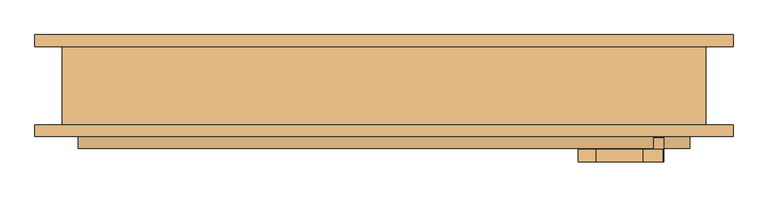
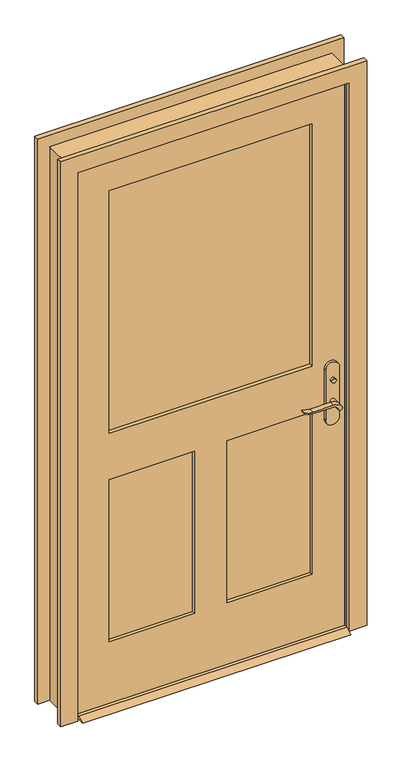
"""IFC4 building model written with IfcOpenShell, lengths in millimetres: door geometry."""

import ifcopenshell
import ifcopenshell.guid

model = None  # the IFC model being written
_history = None  # IfcOwnerHistory: only IFC2X3 demands one
_inside = {}  # id of a spatial element -> (the spatial element, [elements in it])
_under = {}  # id of a project, library or spatial element -> (it, [spatial elements below it])
_declared = {}  # id of a project -> (the project, [libraries it declares])
_typed = {}  # id of a type object -> (the type object, [elements of that type])
_made_of = {}  # id of a material, layer set ... -> (it, [elements and type objects made of it])


def new_model(schema):
    """Start an empty IFC model of exactly this schema.

    Asked for "IFC4X3", IfcOpenShell would pick the latest addendum, in which some entities
    have other attributes; the version numbers below select the first issue.
    IFC2X3 requires an IfcOwnerHistory on every rooted entity: one is made here for all.
    """
    global model, _history
    if schema == "IFC4X3":
        model = ifcopenshell.file(schema_version=(4, 3, 0, 0))
    else:
        model = ifcopenshell.file(schema=schema)
    _inside.clear()
    _under.clear()
    _declared.clear()
    _typed.clear()
    _made_of.clear()
    _history = None
    if model.schema == "IFC2X3":
        org = make("IfcOrganization", Name="unknown")
        user = make(
            "IfcPersonAndOrganization",
            ThePerson=make("IfcPerson", FamilyName="unknown"),
            TheOrganization=org,
        )
        app = make(
            "IfcApplication",
            ApplicationDeveloper=org,
            Version="unknown",
            ApplicationFullName="unknown",
            ApplicationIdentifier="unknown",
        )
        _history = make(
            "IfcOwnerHistory",
            OwningUser=user,
            OwningApplication=app,
            ChangeAction="ADDED",
            CreationDate=0,
        )
    return model


def make(cls, **values):
    """One entity of the class cls with the attributes given. An attribute that is None is left unset."""
    return model.create_entity(
        cls, **{name: value for name, value in values.items() if value is not None}
    )


def rooted(cls, **values):
    """An entity with a GlobalId (a new one), such as an element, a storey or a relation."""
    return make(cls, GlobalId=ifcopenshell.guid.new(), OwnerHistory=_history, **values)


def si_unit(unit_type, name, prefix=None):
    """IfcSIUnit, for example si_unit("LENGTHUNIT", "METRE", prefix="MILLI")."""
    return make("IfcSIUnit", UnitType=unit_type, Prefix=prefix, Name=name)


def assignment(units):
    """IfcUnitAssignment: the units of a project."""
    return None if units is None else make("IfcUnitAssignment", Units=units)


def point(xyz):
    """IfcCartesianPoint."""
    return None if xyz is None else make("IfcCartesianPoint", Coordinates=xyz)


def direction(xyz):
    """IfcDirection."""
    return None if xyz is None else make("IfcDirection", DirectionRatios=xyz)


def frame(location, z_axis=None, x_axis=None):
    """IfcAxis2Placement3D, a coordinate frame: its origin and axes. An axis left out is left unset."""
    return make(
        "IfcAxis2Placement3D",
        Location=point(location),
        Axis=direction(z_axis),
        RefDirection=direction(x_axis),
    )


def frame_2d(location, x_axis=None):
    """IfcAxis2Placement2D, a coordinate frame in the plane: its origin and x axis."""
    return make(
        "IfcAxis2Placement2D", Location=point(location), RefDirection=direction(x_axis)
    )


def origin():
    """The frame at (0, 0, 0) with its axes left unset."""
    return frame((0.0, 0.0, 0.0))


def place(relative_to, where):
    """IfcLocalPlacement: puts the frame where relative to a parent placement (None: the world)."""
    return make(
        "IfcLocalPlacement", PlacementRelTo=relative_to, RelativePlacement=where
    )


def context(
    kind, dimensions, precision=None, world=None, true_north=None, identifier=None
):
    """IfcGeometricRepresentationContext, for example the 3D "Model" context."""
    return make(
        "IfcGeometricRepresentationContext",
        ContextIdentifier=identifier,
        ContextType=kind,
        CoordinateSpaceDimension=dimensions,
        Precision=precision,
        WorldCoordinateSystem=world,
        TrueNorth=true_north,
    )


def project(units=None, contexts=None):
    """IfcProject with its units and contexts."""
    return rooted(
        "IfcProject",
        Name="project",
        RepresentationContexts=contexts,
        UnitsInContext=assignment(units),
    )


def spatial(cls, under=None, at=None, **own):
    """A site, building, storey or space (cls), placed at a placement, below another one or the project."""
    s = rooted(cls, ObjectPlacement=at, **own)
    if under is not None:
        _under.setdefault(under.id(), (under, []))[1].append(s)
    return s


def polyline(points):
    """IfcPolyline through the points."""
    return make("IfcPolyline", Points=[point(p) for p in points])


def circle_curve(where, radius):
    """IfcCircle in the frame where."""
    return make("IfcCircle", Position=where, Radius=radius)


def trimmed(basis, trim1, trim2, sense, master):
    """IfcTrimmedCurve: the piece of a basis curve between two trims."""
    return make(
        "IfcTrimmedCurve",
        BasisCurve=basis,
        Trim1=trim1,
        Trim2=trim2,
        SenseAgreement=sense,
        MasterRepresentation=master,
    )


def segment(curve, same_sense, transition):
    """IfcCompositeCurveSegment."""
    return make(
        "IfcCompositeCurveSegment",
        Transition=transition,
        SameSense=same_sense,
        ParentCurve=curve,
    )


def composite_curve(segments, self_intersect=None):
    """IfcCompositeCurve: segments joined end to end."""
    return make("IfcCompositeCurve", Segments=segments, SelfIntersect=self_intersect)


def outline(outer, holes=None, kind="AREA"):
    """IfcArbitraryClosedProfileDef: a profile drawn as a closed curve; with holes, ...WithVoids."""
    if holes is None:
        return make("IfcArbitraryClosedProfileDef", ProfileType=kind, OuterCurve=outer)
    return make(
        "IfcArbitraryProfileDefWithVoids",
        ProfileType=kind,
        OuterCurve=outer,
        InnerCurves=holes,
    )


def extrude(swept, where, along, depth):
    """IfcExtrudedAreaSolid: the profile swept, set in the frame where, extruded along a direction by depth."""
    return make(
        "IfcExtrudedAreaSolid",
        SweptArea=swept,
        Position=where,
        ExtrudedDirection=direction(along),
        Depth=depth,
    )


def faces_of(points, faces, orient=None, outer=None):
    """IfcFace entities. A face is a list of loops; a loop is a list of indices into points, from 0.

    orient and outer hold one flag for each loop. By default every Orientation is true, the
    first loop of a face is its IfcFaceOuterBound and the others are IfcFaceBound.
    """
    made = []
    for i, loops in enumerate(faces):
        bounds = []
        for j, loop in enumerate(loops):
            is_outer = j == 0 if outer is None else outer[i][j]
            bounds.append(
                make(
                    "IfcFaceOuterBound" if is_outer else "IfcFaceBound",
                    Bound=make("IfcPolyLoop", Polygon=[points[k] for k in loop]),
                    Orientation=True if orient is None else orient[i][j],
                )
            )
        made.append(make("IfcFace", Bounds=bounds))
    return made


def faceted_brep(points, faces, orient=None, outer=None, voids=None):
    """IfcFacetedBrep: a solid bounded by flat faces; with voids (closed shells), ...WithVoids."""
    shared = [point(p) for p in points]
    hull = make("IfcClosedShell", CfsFaces=faces_of(shared, faces, orient, outer))
    if voids is None:
        return make("IfcFacetedBrep", Outer=hull)
    return make(
        "IfcFacetedBrepWithVoids",
        Outer=hull,
        Voids=[
            make(cls, CfsFaces=faces_of(shared, fs, o, b)) for cls, fs, o, b in voids
        ],
    )


def shape(context_of_items, identifier, shape_type, items):
    """IfcShapeRepresentation: the items that make up one representation, for example the "Body"."""
    return make(
        "IfcShapeRepresentation",
        ContextOfItems=context_of_items,
        RepresentationIdentifier=identifier,
        RepresentationType=shape_type,
        Items=items,
    )


def source(mapping_origin, context_of_items, identifier, shape_type, items):
    """IfcRepresentationMap: a shape defined once, which mapped items show again and again."""
    return make(
        "IfcRepresentationMap",
        MappingOrigin=mapping_origin,
        MappedRepresentation=shape(context_of_items, identifier, shape_type, items),
    )


def transform(
    local_origin,
    x_axis=None,
    y_axis=None,
    z_axis=None,
    scale=None,
    scale2=None,
    scale3=None,
    uniform=True,
):
    """IfcCartesianTransformationOperator3D, or its non-uniform kind. x_axis, y_axis, z_axis: its Axis1, 2, 3."""
    if uniform:
        return make(
            "IfcCartesianTransformationOperator3D",
            Axis1=direction(x_axis),
            Axis2=direction(y_axis),
            LocalOrigin=point(local_origin),
            Scale=scale,
            Axis3=direction(z_axis),
        )
    return make(
        "IfcCartesianTransformationOperator3DnonUniform",
        Axis1=direction(x_axis),
        Axis2=direction(y_axis),
        LocalOrigin=point(local_origin),
        Scale=scale,
        Axis3=direction(z_axis),
        Scale2=scale2,
        Scale3=scale3,
    )


def mapped(mapping_source, mapping_target):
    """IfcMappedItem: shows the shape of a source again, moved by a transform."""
    return make(
        "IfcMappedItem", MappingSource=mapping_source, MappingTarget=mapping_target
    )


def made_of(thing, what):
    """Note that an element or type object is made of a material, layer set ...; save() writes the relation."""
    if what is not None:
        _made_of.setdefault(what.id(), (what, []))[1].append(thing)
    return thing


def element(
    cls,
    number,
    at=None,
    inside=None,
    cuts=None,
    type_object=None,
    material=None,
    context=None,
    identifier="Body",
    shape_type=None,
    held_by="IfcProductDefinitionShape",
    body=None,
    shapes=None,
    **own,
):
    """One element of the class cls, such as IfcWall. Its Tag is "e" and its number.

    at: its placement. inside: the storey or other place that contains it. cuts: it is an
    opening in that element (IfcRelVoidsElement). A single representation is given by context,
    identifier, shape_type and body (its items); several are given by shapes. held_by: the class
    of the entity that holds the representations. save() writes the other relations.
    """
    e = rooted(cls, Tag="e%d" % number, ObjectPlacement=at, **own)
    if body is not None:
        shapes = [shape(context, identifier, shape_type, body)]
    if shapes is not None:
        e.Representation = make(held_by, Representations=shapes)
    if inside is not None:
        _inside.setdefault(inside.id(), (inside, []))[1].append(e)
    if cuts is not None:
        rooted(
            "IfcRelVoidsElement", RelatingBuildingElement=cuts, RelatedOpeningElement=e
        )
    if type_object is not None:
        _typed.setdefault(type_object.id(), (type_object, []))[1].append(e)
    return made_of(e, material)


def aggregate(whole, parts):
    """IfcRelAggregates: a whole, such as a stair, and the parts it consists of."""
    return rooted("IfcRelAggregates", RelatingObject=whole, RelatedObjects=parts)


def save(model, path):
    """Write the relations noted so far, then the file.

    IfcRelAggregates (storeys below a building ...), IfcRelContainedInSpatialStructure (elements
    in a storey), IfcRelDefinesByType, IfcRelAssociatesMaterial and IfcRelDeclares: one each for
    every whole, place, type object, material and project.
    """
    for whole, parts in _under.values():
        aggregate(whole, parts)
    for where, things in _inside.values():
        rooted(
            "IfcRelContainedInSpatialStructure",
            RelatedElements=things,
            RelatingStructure=where,
        )
    for kind, things in _typed.values():
        rooted("IfcRelDefinesByType", RelatedObjects=things, RelatingType=kind)
    for what, things in _made_of.values():
        rooted("IfcRelAssociatesMaterial", RelatedObjects=things, RelatingMaterial=what)
    for by, libraries in _declared.values():
        rooted("IfcRelDeclares", RelatingContext=by, RelatedDefinitions=libraries)
    model.write(path)


def door_f2be2632(model_context):
    return source(origin(), model_context, "Body", "SolidModel", [
        extrude(outline(polyline([(-38.1, 12.7), (-12.7, 0.0), (-98.425, 0.0), (-73.025, 12.7), (-38.1, 12.7)])), frame((-495.3, 0.0, 0.0), z_axis=(1.0, 0.0, 0.0), x_axis=(0.0, 1.0, 0.0)), (0.0, 0.0, 1.0), 990.6),
        extrude(outline(polyline([(449.5, -5.4), (449.5, -15.4), (439.5, -15.4), (439.5, -5.4), (449.5, -5.4)])), frame((0.0, 0.0, 981.9), z_axis=(0.0, 0.0, 1.0), x_axis=(1.0, 0.0, 0.0)), (0.0, 0.0, 1.0), 30.0),
        extrude(outline(composite_curve([segment(trimmed(circle_curve(frame_2d((996.9, 444.5)), 8.0), [point((996.9, 436.5))], [point((996.9, 452.5))], False, "CARTESIAN"), True, "CONTINUOUS"), segment(trimmed(circle_curve(frame_2d((996.9, 444.5)), 8.0), [point((996.9, 452.5))], [point((996.9, 436.5))], False, "CARTESIAN"), True, "CONTINUOUS")], self_intersect=False)), frame((0.0, -80.325, 0.0), z_axis=(0.0, 1.0, 0.0), x_axis=(0.0, 0.0, 1.0)), (0.0, 0.0, 1.0), 10.0),
        extrude(outline(composite_curve([segment(trimmed(circle_curve(frame_2d((897.1555521, 420.8324871)), 37.2832219), [point((919.0523287, 451.0081363))], [point((934.4, 419.1325667))], False, "CARTESIAN"), True, "CONTINUOUS"), segment(polyline([(934.4, 419.1325667), (934.4, 342.8564091)]), True, "CONTINUOUS"), segment(trimmed(circle_curve(frame_2d((1017.6850638, 342.9227909)), 83.2850902), [point((934.4, 342.8564091))], [point((939.4, 314.5))], True, "CARTESIAN"), True, "CONTINUOUS"), segment(polyline([(939.4, 314.5), (936.6135558, 314.5)]), True, "CONTINUOUS"), segment(trimmed(circle_curve(frame_2d((986.6709207, 346.4396612)), 59.3791355), [point((936.6135558, 314.5))], [point((927.4, 342.8564091))], False, "CARTESIAN"), True, "CONTINUOUS"), segment(polyline([(927.4, 342.8564091), (927.4, 419.1138099)]), True, "CONTINUOUS"), segment(trimmed(circle_curve(frame_2d((909.2738613, 419.1138099)), 18.1261387), [point((927.4, 419.1138099))], [point((914.4, 436.5))], True, "CARTESIAN"), True, "CONTINUOUS"), segment(trimmed(circle_curve(frame_2d((914.4, 444.5)), 8.0), [point((914.4, 436.5))], [point((919.0523287, 451.0081363))], False, "CARTESIAN"), True, "CONTINUOUS")], self_intersect=False)), frame((0.0, 14.6, 0.0), z_axis=(0.0, 1.0, 0.0), x_axis=(0.0, 0.0, 1.0)), (0.0, 0.0, 1.0), 20.0),
        extrude(outline(composite_curve([segment(trimmed(circle_curve(frame_2d((914.4, 444.5)), 8.0), [point((914.3999903, 436.5))], [point((919.0523287, 451.0081363))], False, "CARTESIAN"), True, "CONTINUOUS"), segment(trimmed(circle_curve(frame_2d((897.1555521, 420.8324871)), 37.2832219), [point((919.0523287, 451.0081363))], [point((934.4, 419.1325667))], False, "CARTESIAN"), True, "CONTINUOUS"), segment(polyline([(934.4, 419.1325667), (934.4, 342.8564091)]), True, "CONTINUOUS"), segment(trimmed(circle_curve(frame_2d((1017.6850638, 342.9227909)), 83.2850902), [point((934.4, 342.8564091))], [point((939.4, 314.5))], True, "CARTESIAN"), True, "CONTINUOUS"), segment(polyline([(939.4, 314.5), (936.6135558, 314.5)]), True, "CONTINUOUS"), segment(trimmed(circle_curve(frame_2d((986.6709207, 346.4396612)), 59.3791355), [point((936.6135558, 314.5))], [point((927.4, 342.8564091))], False, "CARTESIAN"), True, "CONTINUOUS"), segment(polyline([(927.4, 342.8564091), (927.4, 419.1138122)]), True, "CONTINUOUS"), segment(trimmed(circle_curve(frame_2d((909.2738682, 419.1138122)), 18.1261318), [point((927.4, 419.1138122))], [point((914.3999903, 436.5))], True, "CARTESIAN"), True, "CONTINUOUS")], self_intersect=False)), frame((0.0, -120.325, 0.0), z_axis=(0.0, 1.0, 0.0), x_axis=(0.0, 0.0, 1.0)), (0.0, 0.0, 1.0), 20.0),
        extrude(outline(composite_curve([segment(trimmed(circle_curve(frame_2d((914.4, 444.5)), 8.0), [point((914.4, 436.5))], [point((914.4, 452.5))], False, "CARTESIAN"), True, "CONTINUOUS"), segment(trimmed(circle_curve(frame_2d((914.4, 444.5)), 8.0), [point((914.4, 452.5))], [point((914.4, 436.5))], False, "CARTESIAN"), True, "CONTINUOUS")], self_intersect=False)), frame((0.0, -15.4, 0.0), z_axis=(0.0, 1.0, 0.0), x_axis=(0.0, 0.0, 1.0)), (0.0, 0.0, 1.0), 30.0),
        extrude(outline(composite_curve([segment(trimmed(circle_curve(frame_2d((914.4, 444.5)), 8.0), [point((914.4, 436.5))], [point((914.4, 452.5))], False, "CARTESIAN"), True, "CONTINUOUS"), segment(trimmed(circle_curve(frame_2d((914.4, 444.5)), 8.0), [point((914.4, 452.5))], [point((914.4, 436.5))], False, "CARTESIAN"), True, "CONTINUOUS")], self_intersect=False)), frame((0.0, -100.325, 0.0), z_axis=(0.0, 1.0, 0.0), x_axis=(0.0, 0.0, 1.0)), (0.0, 0.0, 1.0), 30.0),
        extrude(outline(composite_curve([segment(polyline([(844.4, 469.5), (1039.4, 469.5)]), True, "CONTINUOUS"), segment(trimmed(circle_curve(frame_2d((1039.4, 444.5)), 25.0), [point((1039.4, 469.5))], [point((1039.4, 419.5))], False, "CARTESIAN"), True, "CONTINUOUS"), segment(polyline([(1039.4, 419.5), (844.4, 419.5)]), True, "CONTINUOUS"), segment(trimmed(circle_curve(frame_2d((844.4, 444.5)), 25.0), [point((844.4, 419.5))], [point((844.4, 469.5))], False, "CARTESIAN"), True, "CONTINUOUS")], self_intersect=False)), frame((0.0, -25.4, 0.0), z_axis=(0.0, 1.0, 0.0), x_axis=(0.0, 0.0, 1.0)), (0.0, 0.0, 1.0), 10.0),
        extrude(outline(composite_curve([segment(polyline([(844.4, 469.5), (1039.4, 469.5)]), True, "CONTINUOUS"), segment(trimmed(circle_curve(frame_2d((1039.4, 444.5)), 25.0), [point((1039.4, 469.5))], [point((1039.4, 419.5))], False, "CARTESIAN"), True, "CONTINUOUS"), segment(polyline([(1039.4, 419.5), (844.4, 419.5)]), True, "CONTINUOUS"), segment(trimmed(circle_curve(frame_2d((844.4, 444.5)), 25.0), [point((844.4, 419.5))], [point((844.4, 469.5))], False, "CARTESIAN"), True, "CONTINUOUS")], self_intersect=False)), frame((0.0, -70.325, 0.0), z_axis=(0.0, 1.0, 0.0), x_axis=(0.0, 0.0, 1.0)), (0.0, 0.0, 1.0), 10.0),
        faceted_brep([(520.7, -60.325, 0.0), (495.3, -60.325, 0.0), (495.3, -25.4, 0.0), (482.6, -25.4, 0.0), (482.6, 9.525, 0.0), (495.3, 9.525, 0.0), (495.3, 66.675, 0.0), (520.7, 66.675, 0.0), (520.7, 66.675, 2159.0), (520.7, -60.325, 2159.0), (495.3, 66.675, 2133.6), (-495.3, 66.675, 2133.6), (-495.3, 66.675, 0.0), (-520.7, 66.675, 0.0), (-520.7, 66.675, 2159.0), (495.3, 9.525, 2133.6), (482.6, 9.525, 2120.9), (-482.6, 9.525, 2120.9), (-482.6, 9.525, 0.0), (-495.3, 9.525, 0.0), (-495.3, 9.525, 2133.6), (482.6, -25.4, 2120.9), (495.3, -25.4, 2133.6), (-495.3, -25.4, 2133.6), (-495.3, -25.4, 0.0), (-482.6, -25.4, 0.0), (-482.6, -25.4, 2120.9), (495.3, -60.325, 2133.6), (-520.7, -60.325, 2159.0), (-520.7, -60.325, 0.0), (-495.3, -60.325, 0.0), (-495.3, -60.325, 2133.6)], [[[0, 1, 2, 3, 4, 5, 6, 7]], [[7, 8, 9, 0]], [[6, 10, 11, 12, 13, 14, 8, 7]], [[5, 15, 10, 6]], [[4, 16, 17, 18, 19, 20, 15, 5]], [[3, 21, 16, 4]], [[2, 22, 23, 24, 25, 26, 21, 3]], [[1, 27, 22, 2]], [[0, 9, 28, 29, 30, 31, 27, 1]], [[8, 14, 28, 9]], [[15, 20, 11, 10]], [[21, 26, 17, 16]], [[27, 31, 23, 22]], [[29, 13, 12, 19, 18, 25, 24, 30]], [[14, 13, 29, 28]], [[20, 19, 12, 11]], [[26, 25, 18, 17]], [[31, 30, 24, 23]]]),
        extrude(outline(polyline([(2133.6, -495.3), (12.7, -495.3), (12.7, 495.3), (2133.6, 495.3), (2133.6, -495.3)]), holes=[polyline([(1066.8, -374.65), (2012.95, -374.65), (2012.95, 374.65), (1066.8, 374.65), (1066.8, -374.65)]), polyline([(885.825, -60.325), (254.0, -60.325), (254.0, -374.65), (885.825, -374.65), (885.825, -60.325)]), polyline([(885.825, 374.65), (254.0, 374.65), (254.0, 60.325), (885.825, 60.325), (885.825, 374.65)])]), frame((0.0, -60.325, 0.0), z_axis=(0.0, 1.0, 0.0), x_axis=(0.0, 0.0, 1.0)), (0.0, 0.0, 1.0), 34.925),
        extrude(outline(polyline([(374.65, -39.37), (374.65, -46.355), (-374.65, -46.355), (-374.65, -39.37), (374.65, -39.37)])), frame((0.0, 0.0, 1066.8), z_axis=(0.0, 0.0, 1.0), x_axis=(1.0, 0.0, 0.0)), (0.0, 0.0, 1.0), 946.15),
        extrude(outline(polyline([(-60.325, -37.0416667), (-60.325, -48.6833333), (-374.65, -48.6833333), (-374.65, -37.0416667), (-60.325, -37.0416667)])), frame((0.0, 0.0, 254.0), z_axis=(0.0, 0.0, 1.0), x_axis=(1.0, 0.0, 0.0)), (0.0, 0.0, 1.0), 631.825),
        extrude(outline(polyline([(374.65, -37.0416667), (374.65, -48.6833333), (60.325, -48.6833333), (60.325, -37.0416667), (374.65, -37.0416667)])), frame((0.0, 0.0, 254.0), z_axis=(0.0, 0.0, 1.0), x_axis=(1.0, 0.0, 0.0)), (0.0, 0.0, 1.0), 631.825),
        extrude(outline(polyline([(0.0, -501.65), (2139.95, -501.65), (2139.95, 501.65), (0.0, 501.65), (0.0, 565.15), (2203.45, 565.15), (2203.45, -565.15), (0.0, -565.15), (0.0, -501.65)])), frame((0.0, -79.375, 0.0), z_axis=(0.0, 1.0, 0.0), x_axis=(0.0, 0.0, 1.0)), (0.0, 0.0, 1.0), 19.05),
        extrude(outline(polyline([(0.0, -501.65), (2139.95, -501.65), (2139.95, 501.65), (0.0, 501.65), (0.0, 565.15), (2203.45, 565.15), (2203.45, -565.15), (0.0, -565.15), (0.0, -501.65)])), frame((0.0, 66.675, 0.0), z_axis=(0.0, 1.0, 0.0), x_axis=(0.0, 0.0, 1.0)), (0.0, 0.0, 1.0), 19.05),
    ])


if __name__ == "__main__":
    model = new_model("IFC4")
    model_context = context("Model", 3, world=origin())
    ifc_project = project(units=[si_unit("LENGTHUNIT", "METRE", prefix="MILLI")], contexts=[model_context])
    site = spatial("IfcSite", under=ifc_project)
    building = spatial("IfcBuilding", under=site)
    placement = place(None, origin())
    door_shape = door_f2be2632(model_context)
    element("IfcDoor", 1, ObjectType="Door-Exterior-Single-Entry-Half Flat Glass-Wood_Clad : 3'3\"*7' Door", at=placement, inside=building, context=model_context, shape_type="MappedRepresentation", body=[
        mapped(door_shape, transform((0.0, 0.0, 0.0), x_axis=(1.0, 0.0, 0.0), y_axis=(0.0, 1.0, 0.0), z_axis=(0.0, 0.0, 1.0))),
    ])
    save(model, "model.ifc")

# Revit data of these elements
# Project information
#   Project Issue Date = "Issue Date"
#   Project Status = "Project Status"
#   Client Name = "Owner"
#   Project Address = "Enter address here"
#   Project Name = "Project Name"
#   Project Number = "Project Number"
# Type "Door-Exterior-Single-Entry-Half Flat Glass-Wood_Clad : 3'3\"*7' Door"
#   Type Mark = "9"
#   Assembly Code = "B2030100"
#   Analytic Construction = "French door, wood frame with single glass"
#   Top Rail = 0' - 4 3/4"
#   Threshold Offset [instance default] = 0' - 0 1/2"
#   Thickness = 0' - 1 3/8"
#   Thermal Resistance (R) = 1.0696 (h·ft²·°F)/BTU
#   Swing Angle [instance default] = 90.00°
#   Stiles = 0' - 4 3/4"
#   Rough Width = 3' - 5"
#   Rough Height = 7' - 1"
#   Lock Rail = 0' - 7 1/8"
#   Height = 7' - 0"
#   Width = 3' - 3"
#   Heat Transfer Coefficient (U) = 0.9350 BTU/(h·ft²·°F)
#   Door Offset [instance default] = 0' - 0"
#   Bottom Rail = 0' - 9 1/2"
#   Threshold [instance default] = yes
#   Function = 1
#   Exterior Trim [instance default] = yes
#   Trim Material = Cherry
#   Threshold Material = Cherry
#   Panel Material = Cherry
#   Glazing = Glass
#   Frame Material = Cherry
#   Door Handle Material = Aluminum
#   Visual Light Transmittance = 0
#   Solar Heat Gain Coefficient = 0
#   Wall Closure = (empty or 0)
#   Construction Type = (empty or 0)
# Element 1 (IfcDoor, "Door-Exterior-Single-Entry-Half Flat Glass-Wood_Clad : 3'3\"*7' Door")
#   Materials on its faces: "Cherry", "Aluminum", "Glass"
# Materials
#   "Cherry": class "Wood", colour RGB 226 177 128, transparency 0, Description = "Prunus Serotina", Cost = 0
#   "Glass": class "Glass", colour RGB 0 128 192, transparency 0.75, Description = "Soda Lime Glass", Cost = 0
#   "Aluminum": class "Metal", colour RGB 247 247 247, transparency 0, Description = "Aluminum 6061", Cost = 0
